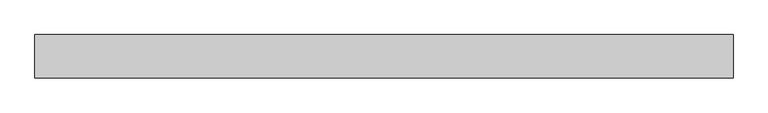
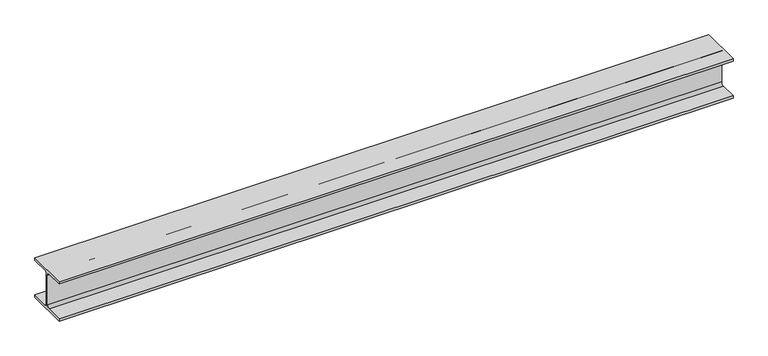
"""IFC4 building model written with IfcOpenShell, lengths in millimetres: beam geometry, 0912_Steel Framing_H-KSD3502 : H_SB_ASB_H-200x200x8x12."""

from ifc_helpers import new_model, si_unit, point, frame, frame_2d, origin, place, context, project, spatial, polyline, circle_curve, trimmed, segment, composite_curve, outline, extrude, source, transform, mapped, element, save


def beam_c0ebad2b(model_context):
    return source(origin(), model_context, "Body", "SweptSolid", [
        extrude(outline(composite_curve([segment(polyline([(100.0, -88.0), (100.0, -100.0), (-100.0, -100.0), (-100.0, -88.0), (-17.0, -88.0)]), True, "CONTINUOUS"), segment(trimmed(circle_curve(frame_2d((-17.0, -75.0)), 13.0), [point((-17.0, -88.0))], [point((-4.0, -75.0))], True, "CARTESIAN"), True, "CONTINUOUS"), segment(polyline([(-4.0, -75.0), (-4.0, 75.0)]), True, "CONTINUOUS"), segment(trimmed(circle_curve(frame_2d((-17.0, 75.0)), 13.0), [point((-4.0, 75.0))], [point((-17.0, 88.0))], True, "CARTESIAN"), True, "CONTINUOUS"), segment(polyline([(-17.0, 88.0), (-100.0, 88.0), (-100.0, 100.0), (100.0, 100.0), (100.0, 88.0), (17.0, 88.0)]), True, "CONTINUOUS"), segment(trimmed(circle_curve(frame_2d((17.0, 75.0)), 13.0), [point((17.0, 88.0))], [point((4.0, 75.0))], True, "CARTESIAN"), True, "CONTINUOUS"), segment(polyline([(4.0, 75.0), (4.0, -75.0)]), True, "CONTINUOUS"), segment(trimmed(circle_curve(frame_2d((17.0, -75.0)), 13.0), [point((4.0, -75.0))], [point((17.0, -88.0))], True, "CARTESIAN"), True, "CONTINUOUS"), segment(polyline([(17.0, -88.0), (100.0, -88.0)]), True, "CONTINUOUS")], self_intersect=False)), frame((-1411.3474079, 0.0, 0.0), z_axis=(1.0, 0.0, 0.0), x_axis=(0.0, 1.0, 0.0)), (0.0, 0.0, 1.0), 3230.5678907),
    ])


if __name__ == "__main__":
    model = new_model("IFC4")
    model_context = context("Model", 3, world=origin())
    ifc_project = project(units=[si_unit("LENGTHUNIT", "METRE", prefix="MILLI")], contexts=[model_context])
    site = spatial("IfcSite", under=ifc_project)
    building = spatial("IfcBuilding", under=site)
    placement = place(None, origin())
    beam_shape = beam_c0ebad2b(model_context)
    element("IfcBeam", 1, ObjectType="0912_Steel Framing_H-KSD3502 : H_SB_ASB_H-200x200x8x12", at=placement, inside=building, context=model_context, shape_type="MappedRepresentation", body=[
        mapped(beam_shape, transform((0.0, 0.0, 0.0), x_axis=(1.0, 0.0, 0.0), y_axis=(0.0, 1.0, 0.0), z_axis=(0.0, 0.0, 1.0))),
    ])
    save(model, "model.ifc")

# Revit data of these elements
# Type "0912_Steel Framing_H-KSD3502 : H_SB_ASB_H-200x200x8x12"
#   H_WM Code_1 = "S01AA002-00001 | Main Steel Structure Fabrication Work | Shelter/Building | Medium Steel - Standard (90KG/M>Weight≥30KG/M) | Material: (   )"
#   H_WM Code_2 = "S03AA028-00001 | Main Steel Structure Erection Work | Shelter/Building | Medium Steel (90KG/M>Weight≥30KG/M) | Material: (   )"
#   H_WM Code_3 = "S01AA010-00001 | Main Steel Structure Fabrication Work | Shelter/Building | Steel Painting/Coating | for Non-Fireproofed Steel Surface, Surface Preparation, Primer, Second & Final Coat | Material: (   )"
#   H_Q'ty Cal Type Tag = "SB-Q2"
#   Width = 20.0 cm
#   Web Thickness = 0.8 cm
#   Web Fillet = 1.3 cm
#   Warping Constant = 141000.0 cm⁶
#   W = 0
#   Torsional Moment of Inertia = 26.2485 cm⁴
#   Section Area = 63.53 cm²
#   Plastic Modulus weak axis = 244.0 cm³
#   Plastic Modulus strong axis = 525.0 cm³
#   Perimeter = 1.16 m²/m
#   Nominal Weight = 49.90 kgf/m
#   Moment of Inertia weak axis = 1600.00 cm⁴
#   Moment of Inertia strong axis = 4720.00 cm⁴
#   Height = 20.0 cm
#   Flange Thickness = 1.2 cm
#   Elastic Modulus weak axis = 160.0 cm³
#   Elastic Modulus strong axis = 472.0 cm³
#   Centroid Vertical = 10.0 cm
#   Centroid Horizontal = 10.0 cm
#   Ix = 47200000
#   Length [instance default] = 1.5240 m
#   Zx = 525000
#   b = 0.2000 m
#   h = 0.2000 m
#   r = 0.0130 m
#   s = 0.0080 m
#   t = 0.0120 m
#   A = 0.006353 m²
#   Structural Material [instance default] = Steel, 45-345
#   Assembly Code = ""
# Element 1 (IfcBeam, "0912_Steel Framing_H-KSD3502 : H_SB_ASB_H-200x200x8x12")
#   Structural Material = none
# Materials
#   "Steel, 45-345": class "Metal", colour RGB 189 187 185, transparency 0, Description = "Steel 345 MPa", Cost = 0
